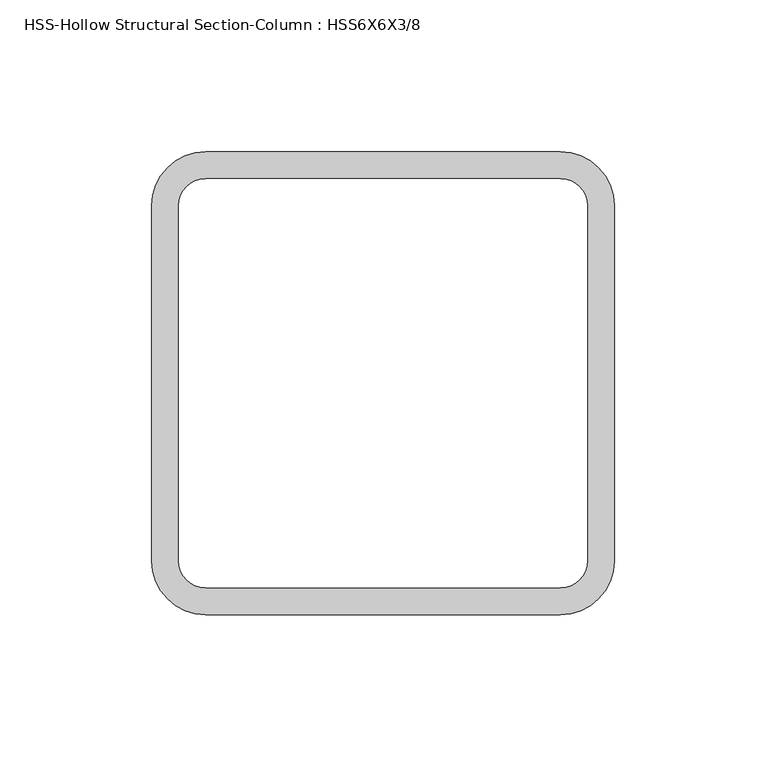
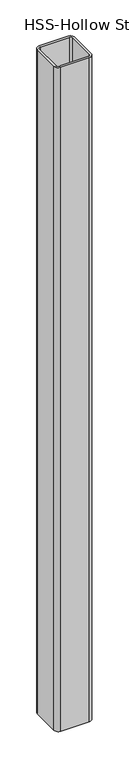
"""IFC4 building model written with IfcOpenShell, lengths in millimetres: column geometry, HSS-Hollow Structural Section-Column : HSS6X6X3/8."""

from ifc_helpers import new_model, si_unit, point, frame, frame_2d, origin, place, context, project, spatial, polyline, circle_curve, trimmed, segment, composite_curve, outline, extrude, source, transform, mapped, element, save


def hss_hollow_structural_section_column_hss6x6x3_8_4dcfe4b9(model_context):
    return source(origin(), model_context, "Body", "SweptSolid", [
        extrude(outline(composite_curve([segment(trimmed(circle_curve(frame_2d((58.4708, 58.4708)), 17.7292), [point((58.4708, 76.2))], [point((76.2, 58.4708))], False, "CARTESIAN"), True, "CONTINUOUS"), segment(polyline([(76.2, 58.4708), (76.2, -58.4708)]), True, "CONTINUOUS"), segment(trimmed(circle_curve(frame_2d((58.4708, -58.4708)), 17.7292), [point((76.2, -58.4708))], [point((58.4708, -76.2))], False, "CARTESIAN"), True, "CONTINUOUS"), segment(polyline([(58.4708, -76.2), (-58.4708, -76.2)]), True, "CONTINUOUS"), segment(trimmed(circle_curve(frame_2d((-58.4708, -58.4708)), 17.7292), [point((-58.4708, -76.2))], [point((-76.2, -58.4708))], False, "CARTESIAN"), True, "CONTINUOUS"), segment(polyline([(-76.2, -58.4708), (-76.2, 58.4708)]), True, "CONTINUOUS"), segment(trimmed(circle_curve(frame_2d((-58.4708, 58.4708)), 17.7292), [point((-76.2, 58.4708))], [point((-58.4708, 76.2))], False, "CARTESIAN"), True, "CONTINUOUS"), segment(polyline([(-58.4708, 76.2), (58.4708, 76.2)]), True, "CONTINUOUS")], self_intersect=False), holes=[composite_curve([segment(polyline([(58.4708, 67.3354), (-58.4708, 67.3354)]), True, "CONTINUOUS"), segment(trimmed(circle_curve(frame_2d((-58.4708, 58.4708)), 8.8646), [point((-58.4708, 67.3354))], [point((-67.3354, 58.4708))], True, "CARTESIAN"), True, "CONTINUOUS"), segment(polyline([(-67.3354, 58.4708), (-67.3354, -58.4708)]), True, "CONTINUOUS"), segment(trimmed(circle_curve(frame_2d((-58.4708, -58.4708)), 8.8646), [point((-67.3354, -58.4708))], [point((-58.4708, -67.3354))], True, "CARTESIAN"), True, "CONTINUOUS"), segment(polyline([(-58.4708, -67.3354), (58.4708, -67.3354)]), True, "CONTINUOUS"), segment(trimmed(circle_curve(frame_2d((58.4708, -58.4708)), 8.8646), [point((58.4708, -67.3354))], [point((67.3354, -58.4708))], True, "CARTESIAN"), True, "CONTINUOUS"), segment(polyline([(67.3354, -58.4708), (67.3354, 58.4708)]), True, "CONTINUOUS"), segment(trimmed(circle_curve(frame_2d((58.4708, 58.4708)), 8.8646), [point((67.3354, 58.4708))], [point((58.4708, 67.3354))], True, "CARTESIAN"), True, "CONTINUOUS")], self_intersect=False)]), frame((0.0, 0.0, 12439.65), z_axis=(0.0, 0.0, 1.0), x_axis=(1.0, 0.0, 0.0)), (0.0, 0.0, 1.0), 2870.2),
    ])


if __name__ == "__main__":
    model = new_model("IFC4")
    model_context = context("Model", 3, world=origin())
    ifc_project = project(units=[si_unit("LENGTHUNIT", "METRE", prefix="MILLI")], contexts=[model_context])
    site = spatial("IfcSite", under=ifc_project)
    building = spatial("IfcBuilding", under=site)
    placement = place(None, origin())
    hss_hollow_structural_section_column_hss6x6x3_8_shape = hss_hollow_structural_section_column_hss6x6x3_8_4dcfe4b9(model_context)
    element("IfcColumn", 1, ObjectType="HSS-Hollow Structural Section-Column : HSS6X6X3/8", at=placement, inside=building, context=model_context, shape_type="MappedRepresentation", body=[
        mapped(hss_hollow_structural_section_column_hss6x6x3_8_shape, transform((0.0, 0.0, 0.0), x_axis=(1.0, 0.0, 0.0), y_axis=(0.0, 1.0, 0.0), z_axis=(0.0, 0.0, 1.0))),
    ])
    save(model, "model.ifc")

# Revit data of these elements
# Type "HSS-Hollow Structural Section-Column : HSS6X6X3/8"
#   Assembly Code = "B10"
#   Shape = "Square"
#   W = 27.4
#   Ht = 0' - 6"
#   b = 0' - 6"
#   kr = 0' - 0.698"
#   t = 0' - 0.349"
#   A = 0.0526389 SF
#   Structural Material [instance default] = Steel ASTM A500, Grade B, Rectangular and Square
# Element 1 (IfcColumn, "HSS-Hollow Structural Section-Column : HSS6X6X3/8")
#   Materials on its faces: "Steel ASTM A500, Grade B, Rectangular and Square"
# Materials
#   "Steel ASTM A500, Grade B, Rectangular and Square": class "Metal", colour RGB 199 199 199, transparency 0, Description = "Carbon steel", Cost = 0
